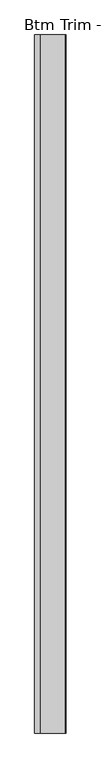
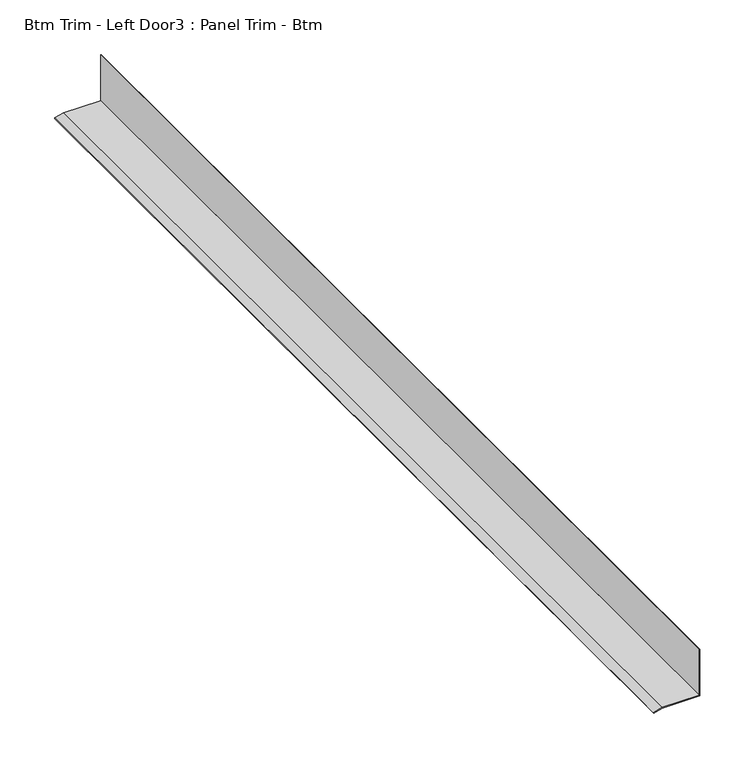
"""IFC4 building model written with IfcOpenShell, lengths in millimetres: proxy geometry, Btm Trim - Left Door3 : Panel Trim - Btm."""

from ifc_helpers import new_model, si_unit, frame, origin, place, context, project, spatial, polyline, outline, extrude, source, transform, mapped, element, save


def btm_trim_left_door3_panel_trim_btm_e3873032(model_context):
    return source(origin(), model_context, "Body", "SweptSolid", [
        extrude(outline(polyline([(50.8, 587326.1141748), (48.3077022, 587316.8127928), (47.5409986, 587317.0182304), (50.00625, 587326.2186739), (50.00625, 587365.8934739), (101.6, 587365.8934739), (101.6, 587365.1060739), (50.8, 587365.1060739), (50.8, 587326.1141748)])), frame((0.0, -535202.3537841, 0.0), z_axis=(0.0, 1.0, 0.0), x_axis=(0.0, 0.0, 1.0)), (0.0, 0.0, 1.0), 1093.7880247),
    ])


if __name__ == "__main__":
    model = new_model("IFC4")
    model_context = context("Model", 3, world=origin())
    ifc_project = project(units=[si_unit("LENGTHUNIT", "METRE", prefix="MILLI")], contexts=[model_context])
    site = spatial("IfcSite", under=ifc_project)
    building = spatial("IfcBuilding", under=site)
    placement = place(None, origin())
    btm_trim_left_door3_panel_trim_btm_shape = btm_trim_left_door3_panel_trim_btm_e3873032(model_context)
    element("IfcBuildingElementProxy", 1, Name="Btm Trim - Left Door3 : Panel Trim - Btm", ObjectType="Btm Trim - Left Door3 : Panel Trim - Btm", at=placement, inside=building, context=model_context, shape_type="MappedRepresentation", body=[
        mapped(btm_trim_left_door3_panel_trim_btm_shape, transform((0.0, 0.0, 0.0), x_axis=(1.0, 0.0, 0.0), y_axis=(0.0, 1.0, 0.0), z_axis=(0.0, 0.0, 1.0))),
    ])
    save(model, "model.ifc")

# Revit data of these elements
# Element 1 (IfcBuildingElementProxy, "Btm Trim - Left Door3 : Panel Trim - Btm")
#   Materials on its faces: "BASE TRIM BY MTL PANEL MFR."
# Materials
#   "BASE TRIM BY MTL PANEL MFR.": class "Generic", colour RGB 239 242 240, transparency 0, Cost = 0
